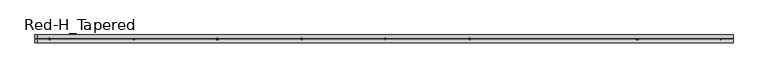
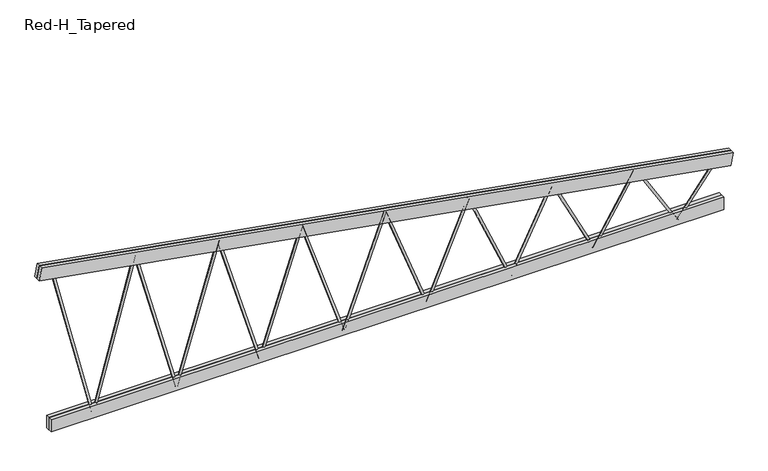
"""IFC4 building model written with IfcOpenShell, lengths in millimetres: beam geometry, Construction_Frames_RedBuilt_Openweb_Red-H_Tapered : Red-H_Tapered."""

import ifcopenshell
import ifcopenshell.guid

model = None  # the IFC model being written
_history = None  # IfcOwnerHistory: only IFC2X3 demands one
_inside = {}  # id of a spatial element -> (the spatial element, [elements in it])
_under = {}  # id of a project, library or spatial element -> (it, [spatial elements below it])
_declared = {}  # id of a project -> (the project, [libraries it declares])
_typed = {}  # id of a type object -> (the type object, [elements of that type])
_made_of = {}  # id of a material, layer set ... -> (it, [elements and type objects made of it])


def new_model(schema):
    """Start an empty IFC model of exactly this schema.

    Asked for "IFC4X3", IfcOpenShell would pick the latest addendum, in which some entities
    have other attributes; the version numbers below select the first issue.
    IFC2X3 requires an IfcOwnerHistory on every rooted entity: one is made here for all.
    """
    global model, _history
    if schema == "IFC4X3":
        model = ifcopenshell.file(schema_version=(4, 3, 0, 0))
    else:
        model = ifcopenshell.file(schema=schema)
    _inside.clear()
    _under.clear()
    _declared.clear()
    _typed.clear()
    _made_of.clear()
    _history = None
    if model.schema == "IFC2X3":
        org = make("IfcOrganization", Name="unknown")
        user = make(
            "IfcPersonAndOrganization",
            ThePerson=make("IfcPerson", FamilyName="unknown"),
            TheOrganization=org,
        )
        app = make(
            "IfcApplication",
            ApplicationDeveloper=org,
            Version="unknown",
            ApplicationFullName="unknown",
            ApplicationIdentifier="unknown",
        )
        _history = make(
            "IfcOwnerHistory",
            OwningUser=user,
            OwningApplication=app,
            ChangeAction="ADDED",
            CreationDate=0,
        )
    return model


def make(cls, **values):
    """One entity of the class cls with the attributes given. An attribute that is None is left unset."""
    return model.create_entity(
        cls, **{name: value for name, value in values.items() if value is not None}
    )


def rooted(cls, **values):
    """An entity with a GlobalId (a new one), such as an element, a storey or a relation."""
    return make(cls, GlobalId=ifcopenshell.guid.new(), OwnerHistory=_history, **values)


def si_unit(unit_type, name, prefix=None):
    """IfcSIUnit, for example si_unit("LENGTHUNIT", "METRE", prefix="MILLI")."""
    return make("IfcSIUnit", UnitType=unit_type, Prefix=prefix, Name=name)


def assignment(units):
    """IfcUnitAssignment: the units of a project."""
    return None if units is None else make("IfcUnitAssignment", Units=units)


def point(xyz):
    """IfcCartesianPoint."""
    return None if xyz is None else make("IfcCartesianPoint", Coordinates=xyz)


def direction(xyz):
    """IfcDirection."""
    return None if xyz is None else make("IfcDirection", DirectionRatios=xyz)


def frame(location, z_axis=None, x_axis=None):
    """IfcAxis2Placement3D, a coordinate frame: its origin and axes. An axis left out is left unset."""
    return make(
        "IfcAxis2Placement3D",
        Location=point(location),
        Axis=direction(z_axis),
        RefDirection=direction(x_axis),
    )


def frame_2d(location, x_axis=None):
    """IfcAxis2Placement2D, a coordinate frame in the plane: its origin and x axis."""
    return make(
        "IfcAxis2Placement2D", Location=point(location), RefDirection=direction(x_axis)
    )


def origin():
    """The frame at (0, 0, 0) with its axes left unset."""
    return frame((0.0, 0.0, 0.0))


def origin_2d():
    """The frame at (0, 0) in the plane with its x axis left unset."""
    return frame_2d((0.0, 0.0))


def place(relative_to, where):
    """IfcLocalPlacement: puts the frame where relative to a parent placement (None: the world)."""
    return make(
        "IfcLocalPlacement", PlacementRelTo=relative_to, RelativePlacement=where
    )


def context(
    kind, dimensions, precision=None, world=None, true_north=None, identifier=None
):
    """IfcGeometricRepresentationContext, for example the 3D "Model" context."""
    return make(
        "IfcGeometricRepresentationContext",
        ContextIdentifier=identifier,
        ContextType=kind,
        CoordinateSpaceDimension=dimensions,
        Precision=precision,
        WorldCoordinateSystem=world,
        TrueNorth=true_north,
    )


def project(units=None, contexts=None):
    """IfcProject with its units and contexts."""
    return rooted(
        "IfcProject",
        Name="project",
        RepresentationContexts=contexts,
        UnitsInContext=assignment(units),
    )


def spatial(cls, under=None, at=None, **own):
    """A site, building, storey or space (cls), placed at a placement, below another one or the project."""
    s = rooted(cls, ObjectPlacement=at, **own)
    if under is not None:
        _under.setdefault(under.id(), (under, []))[1].append(s)
    return s


def polyline(points):
    """IfcPolyline through the points."""
    return make("IfcPolyline", Points=[point(p) for p in points])


def circle_curve(where, radius):
    """IfcCircle in the frame where."""
    return make("IfcCircle", Position=where, Radius=radius)


def trimmed(basis, trim1, trim2, sense, master):
    """IfcTrimmedCurve: the piece of a basis curve between two trims."""
    return make(
        "IfcTrimmedCurve",
        BasisCurve=basis,
        Trim1=trim1,
        Trim2=trim2,
        SenseAgreement=sense,
        MasterRepresentation=master,
    )


def segment(curve, same_sense, transition):
    """IfcCompositeCurveSegment."""
    return make(
        "IfcCompositeCurveSegment",
        Transition=transition,
        SameSense=same_sense,
        ParentCurve=curve,
    )


def composite_curve(segments, self_intersect=None):
    """IfcCompositeCurve: segments joined end to end."""
    return make("IfcCompositeCurve", Segments=segments, SelfIntersect=self_intersect)


def outline(outer, holes=None, kind="AREA"):
    """IfcArbitraryClosedProfileDef: a profile drawn as a closed curve; with holes, ...WithVoids."""
    if holes is None:
        return make("IfcArbitraryClosedProfileDef", ProfileType=kind, OuterCurve=outer)
    return make(
        "IfcArbitraryProfileDefWithVoids",
        ProfileType=kind,
        OuterCurve=outer,
        InnerCurves=holes,
    )


def extrude(swept, where, along, depth):
    """IfcExtrudedAreaSolid: the profile swept, set in the frame where, extruded along a direction by depth."""
    return make(
        "IfcExtrudedAreaSolid",
        SweptArea=swept,
        Position=where,
        ExtrudedDirection=direction(along),
        Depth=depth,
    )


def shape(context_of_items, identifier, shape_type, items):
    """IfcShapeRepresentation: the items that make up one representation, for example the "Body"."""
    return make(
        "IfcShapeRepresentation",
        ContextOfItems=context_of_items,
        RepresentationIdentifier=identifier,
        RepresentationType=shape_type,
        Items=items,
    )


def source(mapping_origin, context_of_items, identifier, shape_type, items):
    """IfcRepresentationMap: a shape defined once, which mapped items show again and again."""
    return make(
        "IfcRepresentationMap",
        MappingOrigin=mapping_origin,
        MappedRepresentation=shape(context_of_items, identifier, shape_type, items),
    )


def transform(
    local_origin,
    x_axis=None,
    y_axis=None,
    z_axis=None,
    scale=None,
    scale2=None,
    scale3=None,
    uniform=True,
):
    """IfcCartesianTransformationOperator3D, or its non-uniform kind. x_axis, y_axis, z_axis: its Axis1, 2, 3."""
    if uniform:
        return make(
            "IfcCartesianTransformationOperator3D",
            Axis1=direction(x_axis),
            Axis2=direction(y_axis),
            LocalOrigin=point(local_origin),
            Scale=scale,
            Axis3=direction(z_axis),
        )
    return make(
        "IfcCartesianTransformationOperator3DnonUniform",
        Axis1=direction(x_axis),
        Axis2=direction(y_axis),
        LocalOrigin=point(local_origin),
        Scale=scale,
        Axis3=direction(z_axis),
        Scale2=scale2,
        Scale3=scale3,
    )


def mapped(mapping_source, mapping_target):
    """IfcMappedItem: shows the shape of a source again, moved by a transform."""
    return make(
        "IfcMappedItem", MappingSource=mapping_source, MappingTarget=mapping_target
    )


def made_of(thing, what):
    """Note that an element or type object is made of a material, layer set ...; save() writes the relation."""
    if what is not None:
        _made_of.setdefault(what.id(), (what, []))[1].append(thing)
    return thing


def element(
    cls,
    number,
    at=None,
    inside=None,
    cuts=None,
    type_object=None,
    material=None,
    context=None,
    identifier="Body",
    shape_type=None,
    held_by="IfcProductDefinitionShape",
    body=None,
    shapes=None,
    **own,
):
    """One element of the class cls, such as IfcWall. Its Tag is "e" and its number.

    at: its placement. inside: the storey or other place that contains it. cuts: it is an
    opening in that element (IfcRelVoidsElement). A single representation is given by context,
    identifier, shape_type and body (its items); several are given by shapes. held_by: the class
    of the entity that holds the representations. save() writes the other relations.
    """
    e = rooted(cls, Tag="e%d" % number, ObjectPlacement=at, **own)
    if body is not None:
        shapes = [shape(context, identifier, shape_type, body)]
    if shapes is not None:
        e.Representation = make(held_by, Representations=shapes)
    if inside is not None:
        _inside.setdefault(inside.id(), (inside, []))[1].append(e)
    if cuts is not None:
        rooted(
            "IfcRelVoidsElement", RelatingBuildingElement=cuts, RelatedOpeningElement=e
        )
    if type_object is not None:
        _typed.setdefault(type_object.id(), (type_object, []))[1].append(e)
    return made_of(e, material)


def aggregate(whole, parts):
    """IfcRelAggregates: a whole, such as a stair, and the parts it consists of."""
    return rooted("IfcRelAggregates", RelatingObject=whole, RelatedObjects=parts)


def save(model, path):
    """Write the relations noted so far, then the file.

    IfcRelAggregates (storeys below a building ...), IfcRelContainedInSpatialStructure (elements
    in a storey), IfcRelDefinesByType, IfcRelAssociatesMaterial and IfcRelDeclares: one each for
    every whole, place, type object, material and project.
    """
    for whole, parts in _under.values():
        aggregate(whole, parts)
    for where, things in _inside.values():
        rooted(
            "IfcRelContainedInSpatialStructure",
            RelatedElements=things,
            RelatingStructure=where,
        )
    for kind, things in _typed.values():
        rooted("IfcRelDefinesByType", RelatedObjects=things, RelatingType=kind)
    for what, things in _made_of.values():
        rooted("IfcRelAssociatesMaterial", RelatedObjects=things, RelatingMaterial=what)
    for by, libraries in _declared.values():
        rooted("IfcRelDeclares", RelatingContext=by, RelatedDefinitions=libraries)
    model.write(path)


def red_h_tapered_85e574f4(model_context):
    return source(origin(), model_context, "Body", "SweptSolid", [
        extrude(outline(composite_curve([segment(trimmed(circle_curve(origin_2d(), 12.7), [point((0.0, 12.6999999))], [point((0.0, -12.7))], False, "CARTESIAN"), True, "CONTINUOUS"), segment(trimmed(circle_curve(origin_2d(), 12.7), [point((0.0, -12.7))], [point((0.0, 12.6999999))], False, "CARTESIAN"), True, "CONTINUOUS")], self_intersect=False)), frame((-446.5835937, 0.0, -367.0101562), z_axis=(-0.3158396035092417, 0.0, 0.9488125973315938), x_axis=(0.0, -1.0, 0.0)), (0.0, 0.0, 1.0), 1413.9569224),
        extrude(outline(composite_curve([segment(trimmed(circle_curve(origin_2d(), 12.7), [point((0.0, -12.7))], [point((0.0, 12.6999999))], False, "CARTESIAN"), True, "CONTINUOUS"), segment(trimmed(circle_curve(origin_2d(), 12.7), [point((0.0, 12.6999999))], [point((0.0, -12.7))], False, "CARTESIAN"), True, "CONTINUOUS")], self_intersect=False)), frame((-1339.7507812, 0.0, -367.0101562), z_axis=(0.31583960350924095, 0.0, 0.9488125973315941), x_axis=(0.0, -1.0, 0.0)), (0.0, 0.0, 1.0), 1413.9569224),
        extrude(outline(composite_curve([segment(trimmed(circle_curve(origin_2d(), 12.7), [point((0.0, 12.7))], [point((0.0, -12.7000001))], False, "CARTESIAN"), True, "CONTINUOUS"), segment(trimmed(circle_curve(origin_2d(), 12.7), [point((0.0, -12.7000001))], [point((0.0, 12.7))], False, "CARTESIAN"), True, "CONTINUOUS")], self_intersect=False)), frame((-1339.7507812, 0.0, -367.0101562), z_axis=(-0.2865629068969148, 0.0, 0.9580614282971579), x_axis=(0.0, -1.0, 0.0)), (0.0, 0.0, 1.0), 1558.4138177),
        extrude(outline(composite_curve([segment(trimmed(circle_curve(origin_2d(), 12.7), [point((0.0, -12.7000001))], [point((0.0, 12.7))], False, "CARTESIAN"), True, "CONTINUOUS"), segment(trimmed(circle_curve(origin_2d(), 12.7), [point((0.0, 12.7))], [point((0.0, -12.7000001))], False, "CARTESIAN"), True, "CONTINUOUS")], self_intersect=False)), frame((-2232.9179687, 0.0, -367.0101562), z_axis=(0.28656290689692226, 0.0, 0.9580614282971557), x_axis=(0.0, -1.0, 0.0)), (0.0, 0.0, 1.0), 1558.4138177),
        extrude(outline(composite_curve([segment(trimmed(circle_curve(origin_2d(), 12.7), [point((0.0, 12.6999999))], [point((0.0, -12.7))], False, "CARTESIAN"), True, "CONTINUOUS"), segment(trimmed(circle_curve(origin_2d(), 12.7), [point((0.0, -12.7))], [point((0.0, 12.6999999))], False, "CARTESIAN"), True, "CONTINUOUS")], self_intersect=False)), frame((-2232.9179687, 0.0, -367.0101562), z_axis=(-0.2620657177651589, 0.0, 0.9650500295695722), x_axis=(0.0, -1.0, 0.0)), (0.0, 0.0, 1.0), 1704.0900945),
        extrude(outline(composite_curve([segment(trimmed(circle_curve(origin_2d(), 12.7), [point((0.0, -12.7))], [point((0.0, 12.6999999))], False, "CARTESIAN"), True, "CONTINUOUS"), segment(trimmed(circle_curve(origin_2d(), 12.7), [point((0.0, 12.6999999))], [point((0.0, -12.7))], False, "CARTESIAN"), True, "CONTINUOUS")], self_intersect=False)), frame((-3126.0851562, 0.0, -367.0101562), z_axis=(0.2620657177651526, 0.0, 0.9650500295695739), x_axis=(0.0, -1.0, 0.0)), (0.0, 0.0, 1.0), 1704.0900945),
        extrude(outline(composite_curve([segment(trimmed(circle_curve(origin_2d(), 12.7), [point((0.0, 12.7))], [point((0.0, -12.7000001))], False, "CARTESIAN"), True, "CONTINUOUS"), segment(trimmed(circle_curve(origin_2d(), 12.7), [point((0.0, -12.7000001))], [point((0.0, 12.7))], False, "CARTESIAN"), True, "CONTINUOUS")], self_intersect=False)), frame((-3126.0851562, 0.0, -367.0101562), z_axis=(-0.24130551579623516, 0.0, 0.9704491991064308), x_axis=(0.0, -1.0, 0.0)), (0.0, 0.0, 1.0), 1850.6978271),
        extrude(outline(composite_curve([segment(trimmed(circle_curve(origin_2d(), 12.7), [point((0.0, 12.7000001))], [point((0.0, -12.6999999))], False, "CARTESIAN"), True, "CONTINUOUS"), segment(trimmed(circle_curve(origin_2d(), 12.7), [point((0.0, -12.6999999))], [point((0.0, 12.7000001))], False, "CARTESIAN"), True, "CONTINUOUS")], self_intersect=False)), frame((3126.0851562, 0.0, -367.0101562), z_axis=(0.607314875287824, 0.0, 0.7944612276594338), x_axis=(0.0, -1.0, 0.0)), (0.0, 0.0, 1.0), 735.3411087),
        extrude(outline(composite_curve([segment(trimmed(circle_curve(origin_2d(), 12.7), [point((0.0, -12.7))], [point((0.0, 12.7))], False, "CARTESIAN"), True, "CONTINUOUS"), segment(trimmed(circle_curve(origin_2d(), 12.7), [point((0.0, 12.7))], [point((0.0, -12.7))], False, "CARTESIAN"), True, "CONTINUOUS")], self_intersect=False)), frame((3126.0851562, 0.0, -367.0101562), z_axis=(-0.5189128854762288, 0.0, 0.8548271271355011), x_axis=(0.0, -1.0, 0.0)), (0.0, 0.0, 1.0), 860.6138068),
        extrude(outline(composite_curve([segment(trimmed(circle_curve(origin_2d(), 12.7), [point((0.0, 12.7000001))], [point((0.0, -12.7))], False, "CARTESIAN"), True, "CONTINUOUS"), segment(trimmed(circle_curve(origin_2d(), 12.7), [point((0.0, -12.7))], [point((0.0, 12.7000001))], False, "CARTESIAN"), True, "CONTINUOUS")], self_intersect=False)), frame((2232.9179687, 0.0, -367.0101562), z_axis=(0.5189128854762283, 0.0, 0.8548271271355016), x_axis=(0.0, -1.0, 0.0)), (0.0, 0.0, 1.0), 860.6138068),
        extrude(outline(composite_curve([segment(trimmed(circle_curve(origin_2d(), 12.7), [point((0.0, -12.7))], [point((0.0, 12.7))], False, "CARTESIAN"), True, "CONTINUOUS"), segment(trimmed(circle_curve(origin_2d(), 12.7), [point((0.0, 12.7))], [point((0.0, -12.7))], False, "CARTESIAN"), True, "CONTINUOUS")], self_intersect=False)), frame((2232.9179687, 0.0, -367.0101562), z_axis=(-0.44963444483494874, 0.0, 0.893212665616631), x_axis=(0.0, -1.0, 0.0)), (0.0, 0.0, 1.0), 993.214819),
        extrude(outline(composite_curve([segment(trimmed(circle_curve(origin_2d(), 12.7), [point((0.0, 12.7000001))], [point((0.0, -12.6999999))], False, "CARTESIAN"), True, "CONTINUOUS"), segment(trimmed(circle_curve(origin_2d(), 12.7), [point((0.0, -12.6999999))], [point((0.0, 12.7000001))], False, "CARTESIAN"), True, "CONTINUOUS")], self_intersect=False)), frame((1339.7507812, 0.0, -367.0101562), z_axis=(0.44963444483494797, 0.0, 0.8932126656166315), x_axis=(0.0, -1.0, 0.0)), (0.0, 0.0, 1.0), 993.214819),
        extrude(outline(composite_curve([segment(trimmed(circle_curve(origin_2d(), 12.7), [point((0.0, -12.7))], [point((0.0, 12.7))], False, "CARTESIAN"), True, "CONTINUOUS"), segment(trimmed(circle_curve(origin_2d(), 12.7), [point((0.0, 12.7))], [point((0.0, -12.7))], False, "CARTESIAN"), True, "CONTINUOUS")], self_intersect=False)), frame((1339.7507812, 0.0, -367.0101562), z_axis=(-0.3950079818502407, 0.0, 0.9186776879159524), x_axis=(0.0, -1.0, 0.0)), (0.0, 0.0, 1.0), 1130.5685309),
        extrude(outline(composite_curve([segment(trimmed(circle_curve(origin_2d(), 12.7), [point((0.0, 12.7))], [point((0.0, -12.7))], False, "CARTESIAN"), True, "CONTINUOUS"), segment(trimmed(circle_curve(origin_2d(), 12.7), [point((0.0, -12.7))], [point((0.0, 12.7))], False, "CARTESIAN"), True, "CONTINUOUS")], self_intersect=False)), frame((446.5835938, 0.0, -367.0101562), z_axis=(0.3950079818502411, 0.0, 0.9186776879159522), x_axis=(0.0, -1.0, 0.0)), (0.0, 0.0, 1.0), 1130.5685309),
        extrude(outline(composite_curve([segment(trimmed(circle_curve(origin_2d(), 12.7), [point((0.0, -12.7000001))], [point((0.0, 12.6999999))], False, "CARTESIAN"), True, "CONTINUOUS"), segment(trimmed(circle_curve(origin_2d(), 12.7), [point((0.0, 12.6999999))], [point((0.0, -12.7000001))], False, "CARTESIAN"), True, "CONTINUOUS")], self_intersect=False)), frame((446.5835938, 0.0, -367.0101562), z_axis=(-0.3513265880589521, 0.0, 0.9362529725041494), x_axis=(0.0, -1.0, 0.0)), (0.0, 0.0, 1.0), 1271.1352028),
        extrude(outline(composite_curve([segment(trimmed(circle_curve(origin_2d(), 12.7), [point((0.0, -12.7))], [point((0.0, 12.7))], False, "CARTESIAN"), True, "CONTINUOUS"), segment(trimmed(circle_curve(origin_2d(), 12.7), [point((0.0, 12.7))], [point((0.0, -12.7))], False, "CARTESIAN"), True, "CONTINUOUS")], self_intersect=False)), frame((-446.5835937, 0.0, -367.0101562), z_axis=(0.3513265880589316, 0.0, 0.9362529725041571), x_axis=(0.0, -1.0, 0.0)), (0.0, 0.0, 1.0), 1271.1352028),
        extrude(outline(polyline([(-3598.06875, -41.275), (-3598.06875, -3.175), (3598.06875, -3.175), (3598.06875, -41.275), (-3598.06875, -41.275)])), frame((0.0, 0.0, -386.0601562), z_axis=(0.0, 0.0, 1.0), x_axis=(1.0, 0.0, 0.0)), (0.0, 0.0, 1.0), 139.7),
        extrude(outline(polyline([(-3598.06875, 3.175), (-3598.06875, 41.275), (3598.06875, 41.275), (3598.06875, 3.175), (-3598.06875, 3.175)])), frame((0.0, 0.0, -386.0601562), z_axis=(0.0, 0.0, 1.0), x_axis=(1.0, 0.0, 0.0)), (0.0, 0.0, 1.0), 139.7),
        extrude(outline(polyline([(0.0, -38.1), (0.0, 0.0), (7509.6947161, 0.0), (7509.6947161, -38.1), (0.0, -38.1)])), frame((-3723.5303312, -3.175, 1368.5927771), z_axis=(0.17080587806736292, 0.0, 0.9853047000890828), x_axis=(0.9853047000890828, 0.0, -0.17080587806736292)), (0.0, 0.0, 1.0), 139.7),
        extrude(outline(polyline([(0.0, -38.1), (0.0, 0.0), (7509.6947161, 0.0), (7509.6947161, -38.1), (0.0, -38.1)])), frame((-3723.5303312, 41.275, 1368.5927771), z_axis=(0.17080587806736292, 0.0, 0.9853047000890828), x_axis=(0.9853047000890828, 0.0, -0.17080587806736292)), (0.0, 0.0, 1.0), 139.7),
    ])


if __name__ == "__main__":
    model = new_model("IFC4")
    model_context = context("Model", 3, world=origin())
    ifc_project = project(units=[si_unit("LENGTHUNIT", "METRE", prefix="MILLI")], contexts=[model_context])
    site = spatial("IfcSite", under=ifc_project)
    building = spatial("IfcBuilding", under=site)
    placement = place(None, origin())
    red_h_tapered_shape = red_h_tapered_85e574f4(model_context)
    element("IfcBeam", 1, ObjectType="Construction_Frames_RedBuilt_Openweb_Red-H_Tapered : Red-H_Tapered", at=placement, inside=building, context=model_context, shape_type="MappedRepresentation", body=[
        mapped(red_h_tapered_shape, transform((0.0, 0.0, 0.0), x_axis=(1.0, 0.0, 0.0), y_axis=(0.0, 1.0, 0.0), z_axis=(0.0, 0.0, 1.0))),
    ])
    save(model, "model.ifc")

# Revit data of these elements
# Type "Construction_Frames_RedBuilt_Openweb_Red-H_Tapered : Red-H_Tapered"
#   Youtube clip = ""
#   Weight Net (Kg) = "0"
#   Webs = "Up to 2\" diameter tubular steel"
#   Uniformat II Description = ""
#   Uniformat II Code = ""
#   Uniclass 2015 Name = "Softwood trusses"
#   Uniclass 2015 Code = "Pr_20_85_90_81"
#   Uniclass 2.0 Description = "Structural Framing Systems"
#   Uniclass 2.0 Code = "SS-15-10-75"
#   Uniclass 1.4 Description = "Trusses"
#   Uniclass 1.4 Code = "L3523"
#   UNSPSC Code = "30103606"
#   Technical description = "http://www.redbuilt.com/reference/literature-and-other-resources"
#   Region South America = "None"
#   Region Oceania = "None"
#   Region North America = "US"
#   Region Middle East = "None"
#   Region Europe = "None"
#   Region Asia = "None"
#   Region Antarctica = "None"
#   Region Africa = "None"
#   QR code = "http://bimobject.com/redbuilt/product/redbuilt-0003"
#   Product url = "http://www.redbuilt.com/products/default.aspx?id=2"
#   Product group = "Wood Trusses"
#   Product family = "Construction"
#   Product data url = "https://bimobject.com/redbuilt/product/redbuilt-0003"
#   Product certification = ""
#   Product SKU = "redbuilt-0003"
#   Product Page URL = "http://www.redbuilt.com/commercial-systems/red-m-red-h-open-web-trusses"
#   Product Guid = "2c5793f2-6ffb-4665-b825-cf90c048e711"
#   Product Documentation Link = "http://www.redbuilt.com/documents/OW_Guide_2017_07_LowRes_wLinks.pdf"
#   OmniClass Description = "Wood Trusses"
#   OmniClass Code = "23-13 35 19 13 17"
#   NBS Reference Description = ""
#   NBS Reference Code = ""
#   Material secondary = "Steel"
#   Material main = "Wood"
#   Masterformat 2014 Description = "Metal-Web Wood Joists"
#   Masterformat 2014 Code = "06 17 36"
#   Manufacturer name = "RedBuilt"
#   Manufacturer country = "United States"
#   Installation instructions = "http://www.redbuilt.com/documents/Installation_Sheets_Open-Web.pdf"
#   IFC Classification = ""
#   EAN code = ""
#   Design country = "United States"
#   Product Information = "http://redbuilt.com/products/default.aspx?id=2"
#   Model = "Red-H-Tapered"
#   Manufacturer URL = "http://redbuilt.com/"
#   Manufacturer = "RedBuilt™"
#   Description = "Open Web Truss"
#   Date of publishing = "8/17/2010"
#   Contact us = "http://redbuilt.com/contact/"
#   Chords = "Double 1½\" x 5½\" MSR lumber"
#   COBIe Type Category = ""
#   Brand url = "http://www.redbuilt.com"
#   BIMobject main category code = "construction"
#   BIMobject main category = "Construction"
#   BIMobject category code = "construction-frames-trusses"
#   BIMobject category = "Frames & Trusses"
#   Web Radius = 0' - 0 1/2"
#   Web Layout Offset Start [instance default] = 0' - 5"
#   Web Layout Offset End [instance default] = 0' - 5"
#   Web Diameter = 0' - 1"
#   TotalLength [instance default] = 20' - 0"
#   Span Minimum = 4' - 0"
#   Span Maximum = 70' - 0"
#   Span Limit [instance default] = 20' - 0"
#   Nominal width = 0' - 0"
#   Nominal height = 0' - 0"
#   Inner Depth Top [instance default] = 0' - 2.76372"
#   Depth Start [instance default] = 6' - 0"
#   Top Chord Length [instance default] = 20' - 1.19701"
#   TC Extension Start Aux [instance default] = 0' - 0"
#   TC Extension End Aux [instance default] = 0' - 0"
#   T-B Chord Length Difference L [instance default] = 0' - 4"
#   T-B Chord Length Difference [instance default] = 0' - 4"
#   Height 2 [instance default] = 6' - 0"
#   Depth Minimum at Wall = 2' - 0"
#   Depth Maximum at Wall = 6' - 0"
#   Depth Lower End [instance default] = 2' - 0"
#   Depth Higher End [instance default] = 6' - 0"
#   Depth End [instance default] = 2' - 0"
#   Depth 2 [instance default] = 2' - 0"
#   Chord Width = 0' - 3 1/4"
#   Chord Thickness = 0' - 1 1/2"
#   Chord Depth = 0' - 5 1/2"
#   Offset Start [instance default] = 0' - 0"
#   TC Extension Start [instance default] = 0' - 0"
#   End Panel = 0' - 5"
#   Offset End [instance default] = 0' - 0"
#   TC Extension End [instance default] = 0' - 0"
#   Length [instance default] = 20' - 0"
#   Angle [instance default] = 5.71059°
#   Span Limit Warning [instance default] = no
#   Edition number = 1
#   Top Bearing Start [instance default] = yes
#   Top Bearing End [instance default] = yes
#   Bottom Bearing Start [instance default] = no
#   Bottom Bearing End [instance default] = no
#   8 Panels [instance default] = yes
#   16 Panels [instance default] = no
#   12 Panels [instance default] = no
#   Web Material = RedBuilt-Steel, Galvanized
#   Clip Material = RedBuilt-Steel, Galvanized
#   Chords Material = RedBuilt-MSR
#   URL = ""
#   Assembly Code = ""
# Element 1 (IfcBeam, "Construction_Frames_RedBuilt_Openweb_Red-H_Tapered : Red-H_Tapered")
#   TotalLength = 24' - 3 5/16"
#   Span Limit = 24' - 3 5/16"
#   Inner Depth Top = 0' - 2.79101"
#   Top Chord Length = 24' - 7.65727"
#   Depth 2 = 4' - 2 1/2"
#   Angle = 9.83468°
#   Materials on its faces: "RedBuilt-Steel, Galvanized", "RedBuilt-MSR"
# Materials
#   "RedBuilt-Steel, Galvanized": class "Metal", colour RGB 164 172 176, transparency 0, Manufacturer = "RedBuilt. LLC", Comments = "Openweb Metal Web", URL = "http://www.redbuilt.com/", Description = "Galvanized steel", Cost = 0
#   "RedBuilt-MSR": class "Wood", colour RGB 213 182 136, transparency 0, Manufacturer = "RedBuilt, LLC", URL = "http://www.redbuilt.com/", Cost = 0
